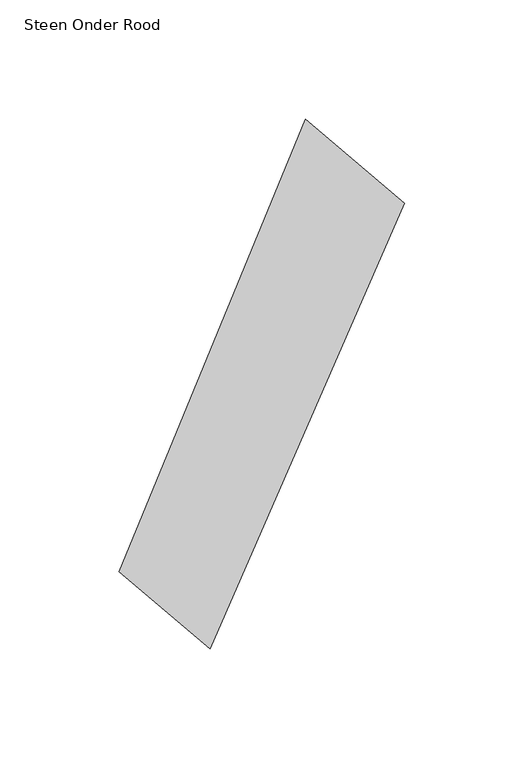
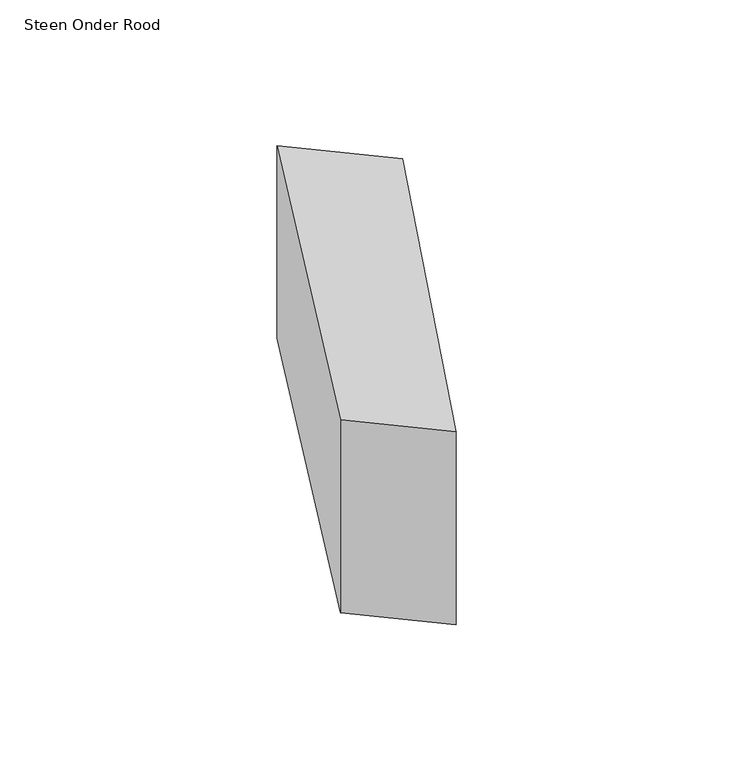
"""IFC4 building model written with IfcOpenShell, lengths in millimetres: proxy geometry, 00_GMA_steen_versie_4 : Steen Onder Rood."""

from ifc_helpers import new_model, si_unit, origin, origin_with_axes, place, context, project, spatial, polyline, outline, extrude, source, transform, mapped, element, save


def steen_onder_rood_1384166a(model_context):
    return source(origin(), model_context, "Body", "SweptSolid", [
        extrude(outline(polyline([(141.5086894, 162.9321077), (59.9700005, -23.8546523), (21.826392, 8.4728148), (100.0647606, 198.0899754), (141.5086894, 162.9321077)])), origin_with_axes(), (0.0, 0.0, 1.0), 100.0),
    ])


if __name__ == "__main__":
    model = new_model("IFC4")
    model_context = context("Model", 3, world=origin())
    ifc_project = project(units=[si_unit("LENGTHUNIT", "METRE", prefix="MILLI")], contexts=[model_context])
    site = spatial("IfcSite", under=ifc_project)
    building = spatial("IfcBuilding", under=site)
    placement = place(None, origin())
    steen_onder_rood_shape = steen_onder_rood_1384166a(model_context)
    element("IfcBuildingElementProxy", 1, Name="00_GMA_steen_versie_4 : Steen Onder Rood", ObjectType="00_GMA_steen_versie_4 : Steen Onder Rood", at=placement, inside=building, context=model_context, shape_type="MappedRepresentation", body=[
        mapped(steen_onder_rood_shape, transform((0.0, 0.0, 0.0), x_axis=(1.0, 0.0, 0.0), y_axis=(0.0, 1.0, 0.0), z_axis=(0.0, 0.0, 1.0))),
    ])
    save(model, "model.ifc")

# Revit data of these elements
# Type "00_GMA_steen_versie_4 : Steen Onder Rood"
#   StootVoegHalfBoven [instance default] = 5 mm
#   StootVoegHalf [instance default] = 5 mm
#   StootVoegBreedteOnder = 10 mm
#   StootVoegBreedteBoven = 10 mm
#   Steendikte = 100 mm
#   LintVoegOnderHalf = 0 mm
#   LintVoegOnder = 0 mm
#   LintVoegBovenHalf = 5 mm
#   LintVoegBoven = 10 mm
#   materiaal = 21_steen_rood
#   MateriaalVoeg = none
#   Default Elevation = 0
# Element 1 (IfcBuildingElementProxy, "00_GMA_steen_versie_4 : Steen Onder Rood")
#   Materials on its faces: "21_steen_rood"
# Materials
#   "21_steen_rood": class "Unassigned", colour RGB 213 111 43, transparency 0, Cost = 0
